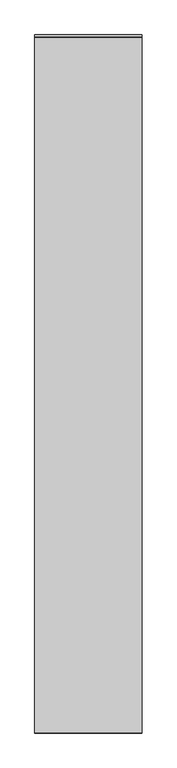
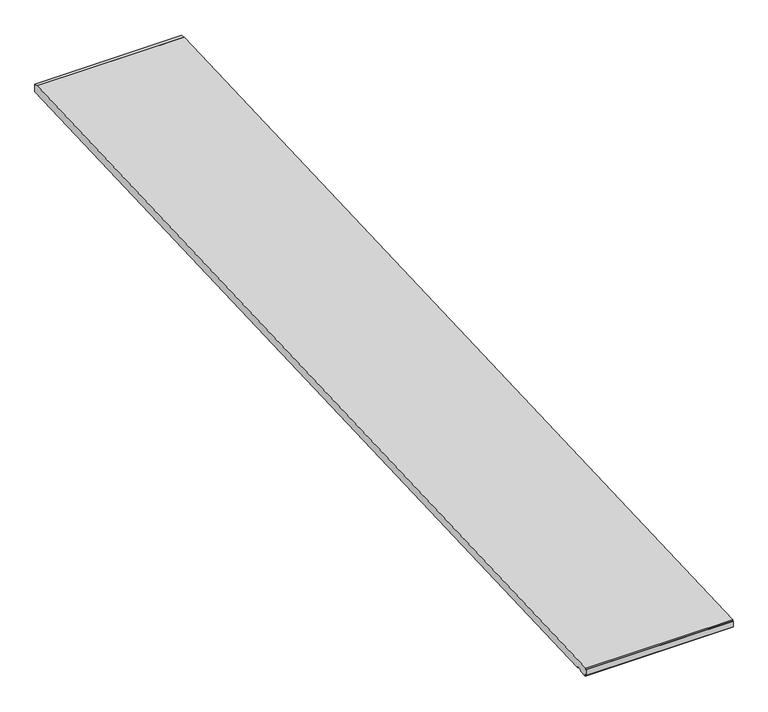
"""IFC4 building model written with IfcOpenShell, lengths in millimetres: proxy geometry, Generic Models 7:Generic Models 1:2:Generic Models 1:2 : Generic Models 7:Generic Models 1:337419:4 : Generic Models 7:Generic Models 1:2:Generic Models 1:2 : Generic Models 7:Generic Models 1:337419:306751."""

from ifc_helpers import new_model, si_unit, frame, origin, place, context, project, spatial, polyline, outline, extrude, source, transform, mapped, element, save


def generic_models_7776ce0e(model_context):
    return source(origin(), model_context, "Body", "SweptSolid", [
        extrude(outline(polyline([(-536698.0341855, 10115.7212544), (-536658.4684898, 10091.947786), (-536560.0695091, 10096.0477436), (-536560.0695091, 9833.4790352), (-567771.0840653, 8533.0200954), (-567783.6188012, 8583.294175), (-567786.1940035, 8585.8693773), (-567923.3188012, 8585.8693773), (-567949.2421701, 8525.596841), (-568212.0117089, 8514.6481102), (-568212.0117089, 8573.8405062), (-568253.3417841, 8572.1184197), (-568253.3417841, 8758.9414091), (-568238.5301636, 8758.9414091), (-568238.5301636, 8801.533922), (-536698.0341855, 10115.7212544)])), frame((591306.0367242, 0.0, 0.0), z_axis=(1.0, 0.0, 0.0), x_axis=(0.0, 1.0, 0.0)), (0.0, 0.0, 1.0), 4876.8),
    ])


if __name__ == "__main__":
    model = new_model("IFC4")
    model_context = context("Model", 3, world=origin())
    ifc_project = project(units=[si_unit("LENGTHUNIT", "METRE", prefix="MILLI")], contexts=[model_context])
    site = spatial("IfcSite", under=ifc_project)
    building = spatial("IfcBuilding", under=site)
    placement = place(None, origin())
    generic_models_shape = generic_models_7776ce0e(model_context)
    element("IfcBuildingElementProxy", 1, Name="Generic Models 7:Generic Models 1:2:Generic Models 1:2 : Generic Models 7:Generic Models 1:337419:4 : Generic Models 7:Generic Models 1:2:Generic Models 1:2 : Generic Models 7:Generic Models 1:337419:306751", ObjectType="Generic Models 7:Generic Models 1:2:Generic Models 1:2 : Generic Models 7:Generic Models 1:337419:4 : Generic Models 7:Generic Models 1:2:Generic Models 1:2 : Generic Models 7:Generic Models 1:337419:306751", at=placement, inside=building, context=model_context, shape_type="MappedRepresentation", body=[
        mapped(generic_models_shape, transform((0.0, 0.0, 0.0), x_axis=(1.0, 0.0, 0.0), y_axis=(0.0, 1.0, 0.0), z_axis=(0.0, 0.0, 1.0))),
    ])
    save(model, "model.ifc")

# Revit data of these elements
# Type "Generic Models 7:Generic Models 1:2:Generic Models 1:2 : Generic Models 7:Generic Models 1:337419:4 : Generic Models 7:Generic Models 1:2:Generic Models 1:2 : Generic Models 7:Generic Models 1:337419:306751"
#   NameOverride = "Generic Models 7:Generic Models 1:2:Generic Models 1:2 : Generic Models 7:Generic Models 1:337419:306751"
#   ObjectTypeOverride = "Generic Models 1:2 : Generic Models 7:Generic Models 1:337419"
#   Reference = "Generic Models 1"
#   Tag = "306751"
# Element 1 (IfcBuildingElementProxy, "Generic Models 7:Generic Models 1:2:Generic Models 1:2 : Generic Models 7:Generic Models 1:337419:4 : Generic Models 7:Generic Models 1:2:Generic Models 1:2 : Generic Models 7:Generic Models 1:337419:306751")
#   Materials on its faces: "SIMPLE SAVER INSULATION WITH LINER - COLOR: WHITE"
# Materials
#   "SIMPLE SAVER INSULATION WITH LINER - COLOR: WHITE": class "Unassigned", colour RGB 219 193 225, transparency 0, Cost = 0
